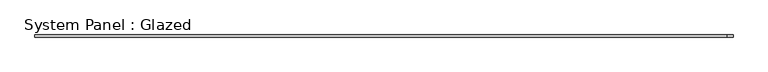
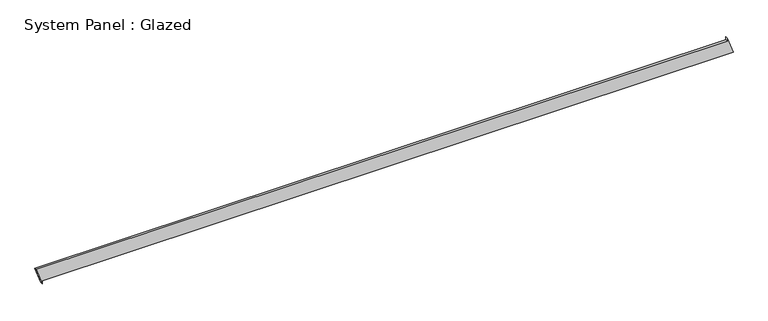
"""IFC4 building model written with IfcOpenShell, lengths in millimetres: plate geometry, System Panel : Glazed."""

from ifc_helpers import new_model, si_unit, frame, origin, place, context, project, spatial, polyline, outline, extrude, source, transform, mapped, element, save


def system_panel_glazed_927418d3(model_context):
    return source(origin(), model_context, "Body", "SweptSolid", [
        extrude(outline(polyline([(0.0, -3957.920533), (35.3553391, -3957.920533), (35.3553391, 4027.1611563), (234.6702265, 3958.2886876), (199.3148875, 3958.2893661), (199.1616377, -4027.1611563), (0.0, -3957.920533)])), frame((0.0, -49.5, 0.0), z_axis=(0.0, 1.0, 0.0), x_axis=(0.0, 0.0, 1.0)), (0.0, 0.0, 1.0), 25.0),
    ])


if __name__ == "__main__":
    model = new_model("IFC4")
    model_context = context("Model", 3, world=origin())
    ifc_project = project(units=[si_unit("LENGTHUNIT", "METRE", prefix="MILLI")], contexts=[model_context])
    site = spatial("IfcSite", under=ifc_project)
    building = spatial("IfcBuilding", under=site)
    placement = place(None, origin())
    system_panel_glazed_shape = system_panel_glazed_927418d3(model_context)
    element("IfcPlate", 1, ObjectType="System Panel : Glazed", at=placement, inside=building, context=model_context, shape_type="MappedRepresentation", body=[
        mapped(system_panel_glazed_shape, transform((0.0, 0.0, 0.0), x_axis=(1.0, 0.0, 0.0), y_axis=(0.0, 1.0, 0.0), z_axis=(0.0, 0.0, 1.0))),
    ])
    save(model, "model.ifc")

# Revit data of these elements
# Element 1 (IfcPlate, "System Panel : Glazed")
#   Materials on its faces: "Glass"
# Materials
#   "Glass": class "Glass", colour RGB 218 227 224, transparency 0.85, Description = "Soda Lime Glass", Cost = 0
